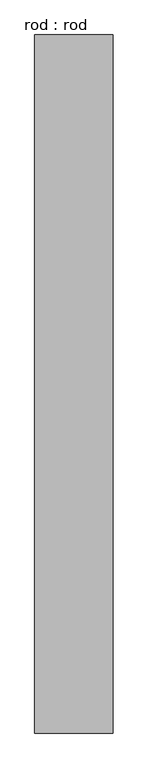
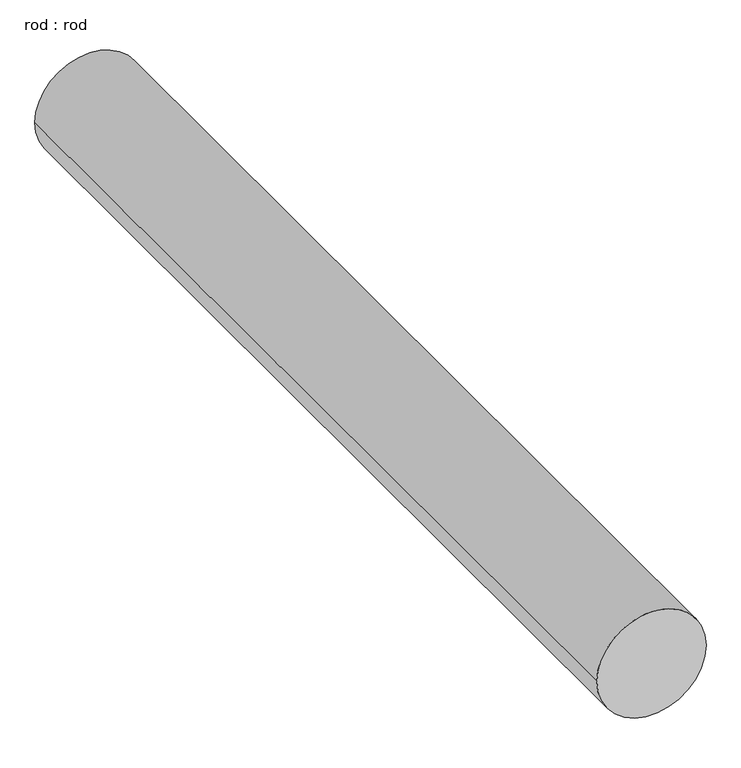
"""IFC4 building model written with IfcOpenShell, lengths in millimetres: proxy geometry, rod : rod."""

from ifc_helpers import new_model, si_unit, point, frame, frame_2d, origin, place, context, project, spatial, circle_curve, trimmed, segment, composite_curve, outline, extrude, source, transform, mapped, element, save


def rod_rod_1b6db2cf(model_context):
    return source(origin(), model_context, "Body", "SweptSolid", [
        extrude(outline(composite_curve([segment(trimmed(circle_curve(frame_2d((0.0108462, 0.0)), 200.0), [point((0.0108462, 200.0))], [point((0.0108462, -200.0))], False, "CARTESIAN"), True, "CONTINUOUS"), segment(trimmed(circle_curve(frame_2d((0.0108462, 0.0)), 200.0), [point((0.0108462, -200.0))], [point((0.0108462, 200.0))], False, "CARTESIAN"), True, "CONTINUOUS")], self_intersect=False)), frame((0.0, 2308.8000439, 0.0), z_axis=(0.0, 1.0, 0.0), x_axis=(0.0, 0.0, 1.0)), (0.0, 0.0, 1.0), 3567.8571429),
    ])


if __name__ == "__main__":
    model = new_model("IFC4")
    model_context = context("Model", 3, world=origin())
    ifc_project = project(units=[si_unit("LENGTHUNIT", "METRE", prefix="MILLI")], contexts=[model_context])
    site = spatial("IfcSite", under=ifc_project)
    building = spatial("IfcBuilding", under=site)
    placement = place(None, origin())
    rod_rod_shape = rod_rod_1b6db2cf(model_context)
    element("IfcBuildingElementProxy", 1, Name="rod : rod", ObjectType="rod : rod", at=placement, inside=building, context=model_context, shape_type="MappedRepresentation", body=[
        mapped(rod_rod_shape, transform((0.0, 0.0, 0.0), x_axis=(1.0, 0.0, 0.0), y_axis=(0.0, 1.0, 0.0), z_axis=(0.0, 0.0, 1.0))),
    ])
    save(model, "model.ifc")

# Revit data of these elements
# Type "rod : rod"
#   Default Elevation = 0
